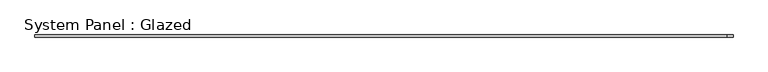
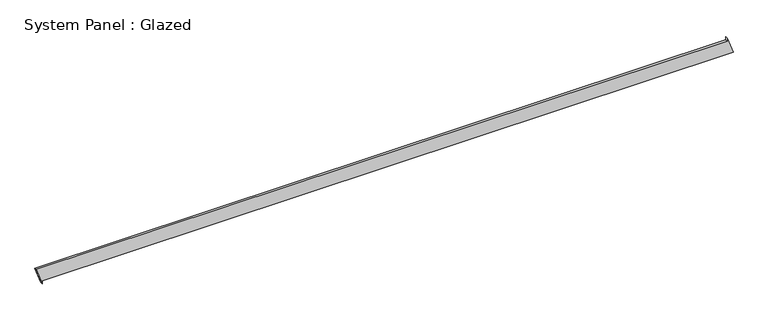
"""IFC4 building model written with IfcOpenShell, lengths in millimetres: plate geometry, System Panel : Glazed."""

import ifcopenshell
import ifcopenshell.guid

model = None  # the IFC model being written
_history = None  # IfcOwnerHistory: only IFC2X3 demands one
_inside = {}  # id of a spatial element -> (the spatial element, [elements in it])
_under = {}  # id of a project, library or spatial element -> (it, [spatial elements below it])
_declared = {}  # id of a project -> (the project, [libraries it declares])
_typed = {}  # id of a type object -> (the type object, [elements of that type])
_made_of = {}  # id of a material, layer set ... -> (it, [elements and type objects made of it])


def new_model(schema):
    """Start an empty IFC model of exactly this schema.

    Asked for "IFC4X3", IfcOpenShell would pick the latest addendum, in which some entities
    have other attributes; the version numbers below select the first issue.
    IFC2X3 requires an IfcOwnerHistory on every rooted entity: one is made here for all.
    """
    global model, _history
    if schema == "IFC4X3":
        model = ifcopenshell.file(schema_version=(4, 3, 0, 0))
    else:
        model = ifcopenshell.file(schema=schema)
    _inside.clear()
    _under.clear()
    _declared.clear()
    _typed.clear()
    _made_of.clear()
    _history = None
    if model.schema == "IFC2X3":
        org = make("IfcOrganization", Name="unknown")
        user = make(
            "IfcPersonAndOrganization",
            ThePerson=make("IfcPerson", FamilyName="unknown"),
            TheOrganization=org,
        )
        app = make(
            "IfcApplication",
            ApplicationDeveloper=org,
            Version="unknown",
            ApplicationFullName="unknown",
            ApplicationIdentifier="unknown",
        )
        _history = make(
            "IfcOwnerHistory",
            OwningUser=user,
            OwningApplication=app,
            ChangeAction="ADDED",
            CreationDate=0,
        )
    return model


def make(cls, **values):
    """One entity of the class cls with the attributes given. An attribute that is None is left unset."""
    return model.create_entity(
        cls, **{name: value for name, value in values.items() if value is not None}
    )


def rooted(cls, **values):
    """An entity with a GlobalId (a new one), such as an element, a storey or a relation."""
    return make(cls, GlobalId=ifcopenshell.guid.new(), OwnerHistory=_history, **values)


def si_unit(unit_type, name, prefix=None):
    """IfcSIUnit, for example si_unit("LENGTHUNIT", "METRE", prefix="MILLI")."""
    return make("IfcSIUnit", UnitType=unit_type, Prefix=prefix, Name=name)


def assignment(units):
    """IfcUnitAssignment: the units of a project."""
    return None if units is None else make("IfcUnitAssignment", Units=units)


def point(xyz):
    """IfcCartesianPoint."""
    return None if xyz is None else make("IfcCartesianPoint", Coordinates=xyz)


def direction(xyz):
    """IfcDirection."""
    return None if xyz is None else make("IfcDirection", DirectionRatios=xyz)


def frame(location, z_axis=None, x_axis=None):
    """IfcAxis2Placement3D, a coordinate frame: its origin and axes. An axis left out is left unset."""
    return make(
        "IfcAxis2Placement3D",
        Location=point(location),
        Axis=direction(z_axis),
        RefDirection=direction(x_axis),
    )


def origin():
    """The frame at (0, 0, 0) with its axes left unset."""
    return frame((0.0, 0.0, 0.0))


def place(relative_to, where):
    """IfcLocalPlacement: puts the frame where relative to a parent placement (None: the world)."""
    return make(
        "IfcLocalPlacement", PlacementRelTo=relative_to, RelativePlacement=where
    )


def context(
    kind, dimensions, precision=None, world=None, true_north=None, identifier=None
):
    """IfcGeometricRepresentationContext, for example the 3D "Model" context."""
    return make(
        "IfcGeometricRepresentationContext",
        ContextIdentifier=identifier,
        ContextType=kind,
        CoordinateSpaceDimension=dimensions,
        Precision=precision,
        WorldCoordinateSystem=world,
        TrueNorth=true_north,
    )


def project(units=None, contexts=None):
    """IfcProject with its units and contexts."""
    return rooted(
        "IfcProject",
        Name="project",
        RepresentationContexts=contexts,
        UnitsInContext=assignment(units),
    )


def spatial(cls, under=None, at=None, **own):
    """A site, building, storey or space (cls), placed at a placement, below another one or the project."""
    s = rooted(cls, ObjectPlacement=at, **own)
    if under is not None:
        _under.setdefault(under.id(), (under, []))[1].append(s)
    return s


def polyline(points):
    """IfcPolyline through the points."""
    return make("IfcPolyline", Points=[point(p) for p in points])


def outline(outer, holes=None, kind="AREA"):
    """IfcArbitraryClosedProfileDef: a profile drawn as a closed curve; with holes, ...WithVoids."""
    if holes is None:
        return make("IfcArbitraryClosedProfileDef", ProfileType=kind, OuterCurve=outer)
    return make(
        "IfcArbitraryProfileDefWithVoids",
        ProfileType=kind,
        OuterCurve=outer,
        InnerCurves=holes,
    )


def extrude(swept, where, along, depth):
    """IfcExtrudedAreaSolid: the profile swept, set in the frame where, extruded along a direction by depth."""
    return make(
        "IfcExtrudedAreaSolid",
        SweptArea=swept,
        Position=where,
        ExtrudedDirection=direction(along),
        Depth=depth,
    )


def shape(context_of_items, identifier, shape_type, items):
    """IfcShapeRepresentation: the items that make up one representation, for example the "Body"."""
    return make(
        "IfcShapeRepresentation",
        ContextOfItems=context_of_items,
        RepresentationIdentifier=identifier,
        RepresentationType=shape_type,
        Items=items,
    )


def source(mapping_origin, context_of_items, identifier, shape_type, items):
    """IfcRepresentationMap: a shape defined once, which mapped items show again and again."""
    return make(
        "IfcRepresentationMap",
        MappingOrigin=mapping_origin,
        MappedRepresentation=shape(context_of_items, identifier, shape_type, items),
    )


def transform(
    local_origin,
    x_axis=None,
    y_axis=None,
    z_axis=None,
    scale=None,
    scale2=None,
    scale3=None,
    uniform=True,
):
    """IfcCartesianTransformationOperator3D, or its non-uniform kind. x_axis, y_axis, z_axis: its Axis1, 2, 3."""
    if uniform:
        return make(
            "IfcCartesianTransformationOperator3D",
            Axis1=direction(x_axis),
            Axis2=direction(y_axis),
            LocalOrigin=point(local_origin),
            Scale=scale,
            Axis3=direction(z_axis),
        )
    return make(
        "IfcCartesianTransformationOperator3DnonUniform",
        Axis1=direction(x_axis),
        Axis2=direction(y_axis),
        LocalOrigin=point(local_origin),
        Scale=scale,
        Axis3=direction(z_axis),
        Scale2=scale2,
        Scale3=scale3,
    )


def mapped(mapping_source, mapping_target):
    """IfcMappedItem: shows the shape of a source again, moved by a transform."""
    return make(
        "IfcMappedItem", MappingSource=mapping_source, MappingTarget=mapping_target
    )


def made_of(thing, what):
    """Note that an element or type object is made of a material, layer set ...; save() writes the relation."""
    if what is not None:
        _made_of.setdefault(what.id(), (what, []))[1].append(thing)
    return thing


def element(
    cls,
    number,
    at=None,
    inside=None,
    cuts=None,
    type_object=None,
    material=None,
    context=None,
    identifier="Body",
    shape_type=None,
    held_by="IfcProductDefinitionShape",
    body=None,
    shapes=None,
    **own,
):
    """One element of the class cls, such as IfcWall. Its Tag is "e" and its number.

    at: its placement. inside: the storey or other place that contains it. cuts: it is an
    opening in that element (IfcRelVoidsElement). A single representation is given by context,
    identifier, shape_type and body (its items); several are given by shapes. held_by: the class
    of the entity that holds the representations. save() writes the other relations.
    """
    e = rooted(cls, Tag="e%d" % number, ObjectPlacement=at, **own)
    if body is not None:
        shapes = [shape(context, identifier, shape_type, body)]
    if shapes is not None:
        e.Representation = make(held_by, Representations=shapes)
    if inside is not None:
        _inside.setdefault(inside.id(), (inside, []))[1].append(e)
    if cuts is not None:
        rooted(
            "IfcRelVoidsElement", RelatingBuildingElement=cuts, RelatedOpeningElement=e
        )
    if type_object is not None:
        _typed.setdefault(type_object.id(), (type_object, []))[1].append(e)
    return made_of(e, material)


def aggregate(whole, parts):
    """IfcRelAggregates: a whole, such as a stair, and the parts it consists of."""
    return rooted("IfcRelAggregates", RelatingObject=whole, RelatedObjects=parts)


def save(model, path):
    """Write the relations noted so far, then the file.

    IfcRelAggregates (storeys below a building ...), IfcRelContainedInSpatialStructure (elements
    in a storey), IfcRelDefinesByType, IfcRelAssociatesMaterial and IfcRelDeclares: one each for
    every whole, place, type object, material and project.
    """
    for whole, parts in _under.values():
        aggregate(whole, parts)
    for where, things in _inside.values():
        rooted(
            "IfcRelContainedInSpatialStructure",
            RelatedElements=things,
            RelatingStructure=where,
        )
    for kind, things in _typed.values():
        rooted("IfcRelDefinesByType", RelatedObjects=things, RelatingType=kind)
    for what, things in _made_of.values():
        rooted("IfcRelAssociatesMaterial", RelatedObjects=things, RelatingMaterial=what)
    for by, libraries in _declared.values():
        rooted("IfcRelDeclares", RelatingContext=by, RelatedDefinitions=libraries)
    model.write(path)


def system_panel_glazed_e03a77ac(model_context):
    return source(origin(), model_context, "Body", "SweptSolid", [
        extrude(outline(polyline([(0.0, -3958.6046047), (35.3553391, -3958.6046047), (35.3553391, 4028.4340057), (234.3037327, 3958.6865343), (198.9483937, 3958.6866872), (198.9138478, -4028.4340057), (0.0, -3958.6046047)])), frame((0.0, -49.5, 0.0), z_axis=(0.0, 1.0, 0.0), x_axis=(0.0, 0.0, 1.0)), (0.0, 0.0, 1.0), 25.0),
    ])


if __name__ == "__main__":
    model = new_model("IFC4")
    model_context = context("Model", 3, world=origin())
    ifc_project = project(units=[si_unit("LENGTHUNIT", "METRE", prefix="MILLI")], contexts=[model_context])
    site = spatial("IfcSite", under=ifc_project)
    building = spatial("IfcBuilding", under=site)
    placement = place(None, origin())
    system_panel_glazed_shape = system_panel_glazed_e03a77ac(model_context)
    element("IfcPlate", 1, ObjectType="System Panel : Glazed", at=placement, inside=building, context=model_context, shape_type="MappedRepresentation", body=[
        mapped(system_panel_glazed_shape, transform((0.0, 0.0, 0.0), x_axis=(1.0, 0.0, 0.0), y_axis=(0.0, 1.0, 0.0), z_axis=(0.0, 0.0, 1.0))),
    ])
    save(model, "model.ifc")

# Revit data of these elements
# Element 1 (IfcPlate, "System Panel : Glazed")
#   Materials on its faces: "Glass"
# Materials
#   "Glass": class "Glass", colour RGB 218 227 224, transparency 0.85, Description = "Soda Lime Glass", Cost = 0
